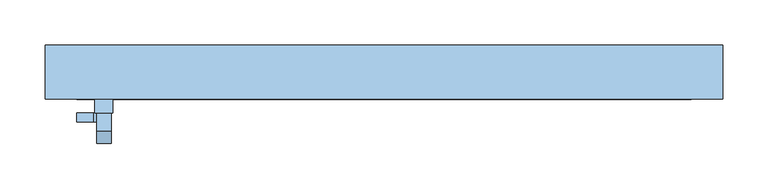
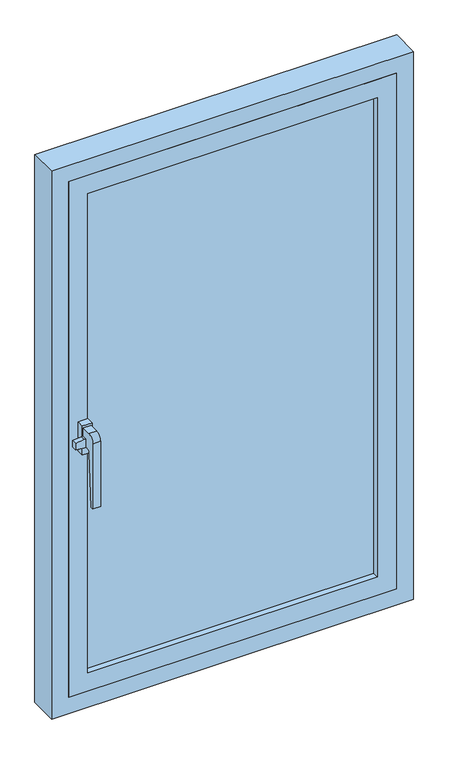
"""IFC4 building model written with IfcOpenShell, lengths in millimetres: window geometry, Inclinar e virar janela - 1 Painel : Inclinar e virar janela - 1 Painel 0,75m."""

from ifc_helpers import new_model, si_unit, point, frame, frame_2d, origin, place, context, project, spatial, polyline, circle_curve, trimmed, segment, composite_curve, outline, extrude, source, transform, mapped, element, save


def window_9ba87819(model_context):
    return source(origin(), model_context, "Body", "SweptSolid", [
        extrude(outline(composite_curve([segment(polyline([(-95.0, 1259.0), (-95.0, 1241.0), (-100.9630874, 1241.0)]), True, "CONTINUOUS"), segment(trimmed(circle_curve(frame_2d((-100.9630874, 1234.9630874)), 6.0369126), [point((-100.9630874, 1241.0))], [point((-106.9888756, 1235.3294081))], True, "CARTESIAN"), True, "CONTINUOUS"), segment(polyline([(-106.9888756, 1235.3294081), (-114.0, 1120.0), (-119.0, 1120.0), (-119.0, 1263.0)]), True, "CONTINUOUS"), segment(trimmed(circle_curve(frame_2d((-105.0, 1263.0)), 14.0), [point((-119.0, 1263.0))], [point((-105.0, 1277.0))], False, "CARTESIAN"), True, "CONTINUOUS"), segment(polyline([(-105.0, 1277.0), (-85.0, 1277.0), (-85.0, 1259.0), (-95.0, 1259.0)]), True, "CONTINUOUS")], self_intersect=False)), frame((-318.0, 0.0, 0.0), z_axis=(1.0, 0.0, 0.0), x_axis=(0.0, 1.0, 0.0)), (0.0, 0.0, 1.0), 16.0),
        extrude(outline(polyline([(1259.0, -302.0), (1259.0, -321.9864015), (1257.0348924, -340.0), (1243.0157191, -340.0), (1241.0, -321.9864015), (1241.0, -302.0), (1259.0, -302.0)])), frame((0.0, -95.0, 0.0), z_axis=(0.0, 1.0, 0.0), x_axis=(0.0, 0.0, 1.0)), (0.0, 0.0, 1.0), 10.0),
        extrude(outline(polyline([(-320.0, -85.0), (-320.0, -70.0), (-300.0, -70.0), (-300.0, -85.0), (-320.0, -85.0)])), frame((0.0, 0.0, 1218.0), z_axis=(0.0, 0.0, 1.0), x_axis=(1.0, 0.0, 0.0)), (0.0, 0.0, 1.0), 64.0),
        extrude(outline(polyline([(300.0, -43.0), (300.0, -57.0), (-300.0, -57.0), (-300.0, -43.0), (300.0, -43.0)])), frame((0.0, 0.0, 725.0), z_axis=(0.0, 0.0, 1.0), x_axis=(1.0, 0.0, 0.0)), (0.0, 0.0, 1.0), 1050.0),
        extrude(outline(polyline([(685.0, -340.0), (685.0, 340.0), (1815.0, 340.0), (1815.0, -340.0), (685.0, -340.0)]), holes=[polyline([(1775.0, -300.0), (1775.0, 300.0), (725.0, 300.0), (725.0, -300.0), (1775.0, -300.0)])]), frame((0.0, -70.0, 0.0), z_axis=(0.0, 1.0, 0.0), x_axis=(0.0, 0.0, 1.0)), (0.0, 0.0, 1.0), 40.0),
        extrude(outline(polyline([(650.0, -375.0), (650.0, 375.0), (1850.0, 375.0), (1850.0, -375.0), (650.0, -375.0)]), holes=[polyline([(1815.0, -340.0), (1815.0, 340.0), (685.0, 340.0), (685.0, -340.0), (1815.0, -340.0)])]), frame((0.0, -70.0, 0.0), z_axis=(0.0, 1.0, 0.0), x_axis=(0.0, 0.0, 1.0)), (0.0, 0.0, 1.0), 60.0),
    ])


if __name__ == "__main__":
    model = new_model("IFC4")
    model_context = context("Model", 3, world=origin())
    ifc_project = project(units=[si_unit("LENGTHUNIT", "METRE", prefix="MILLI")], contexts=[model_context])
    site = spatial("IfcSite", under=ifc_project)
    building = spatial("IfcBuilding", under=site)
    placement = place(None, origin())
    window_shape = window_9ba87819(model_context)
    element("IfcWindow", 1, ObjectType="Inclinar e virar janela - 1 Painel : Inclinar e virar janela - 1 Painel 0,75m", at=placement, inside=building, context=model_context, shape_type="MappedRepresentation", body=[
        mapped(window_shape, transform((0.0, 0.0, 0.0), x_axis=(1.0, 0.0, 0.0), y_axis=(0.0, 1.0, 0.0), z_axis=(0.0, 0.0, 1.0))),
    ])
    save(model, "model.ifc")

# Revit data of these elements
# Type "Inclinar e virar janela - 1 Painel : Inclinar e virar janela - 1 Painel 0,75m"
#   Type Mark = "EF30"
#   Construction Type Id = "SGL"
#   Analytic Construction = "Janelas grandes envidraçadas únicas"
#   W1 = 0.680 m
#   Visual Light Transmittance = 0.9
#   Solar Heat Gain Coefficient = 0.86
#   Rough Width = 0.750 m
#   Rough Height = 1.200 m
#   Largura da moldura do painel = 0.040 m
#   Espessura da moldura do painel = 0.040 m
#   Height = 1.200 m
#   Heat Transfer Coefficient (U) = 5.5617 W/(m²·K)
#   H1 = 1.130 m
#   Largura da estrutura = 0.035 m
#   Espessura da moldura = 0.060 m
#   Altura-padrão do peitoril = 0.650 m
#   Width = 0.750 m
#   Define Thermal Properties by = 1
#   Material do puxador = none
#   Vidro = none
#   Material da moldura = none
#   Wall Closure = (empty or 0)
# Element 1 (IfcWindow, "Inclinar e virar janela - 1 Painel : Inclinar e virar janela - 1 Painel 0,75m")
#   Materials on its faces: "Glass"
# Materials
#   "Glass": class "Glass", colour RGB 0 128 192, transparency 0.75, Description = "Soda Lime Glass", Cost = 0
